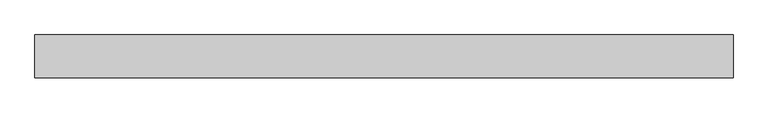
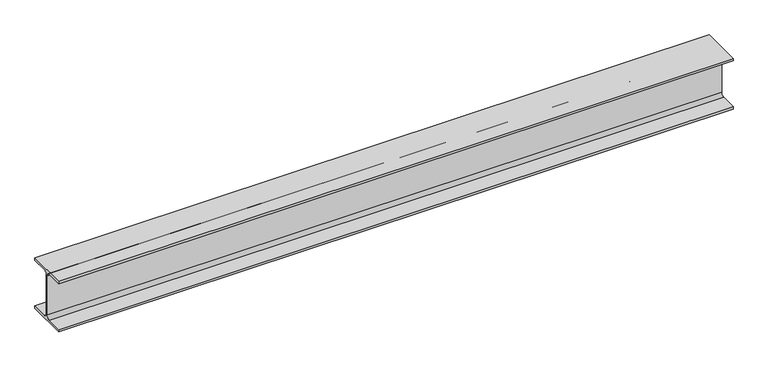
"""IFC4 building model written with IfcOpenShell, lengths in millimetres: beam geometry, 0912_Steel Framing_H-KSD3502 : H_SB_ASB_H-194x150x6x9."""

import ifcopenshell
import ifcopenshell.guid

model = None  # the IFC model being written
_history = None  # IfcOwnerHistory: only IFC2X3 demands one
_inside = {}  # id of a spatial element -> (the spatial element, [elements in it])
_under = {}  # id of a project, library or spatial element -> (it, [spatial elements below it])
_declared = {}  # id of a project -> (the project, [libraries it declares])
_typed = {}  # id of a type object -> (the type object, [elements of that type])
_made_of = {}  # id of a material, layer set ... -> (it, [elements and type objects made of it])


def new_model(schema):
    """Start an empty IFC model of exactly this schema.

    Asked for "IFC4X3", IfcOpenShell would pick the latest addendum, in which some entities
    have other attributes; the version numbers below select the first issue.
    IFC2X3 requires an IfcOwnerHistory on every rooted entity: one is made here for all.
    """
    global model, _history
    if schema == "IFC4X3":
        model = ifcopenshell.file(schema_version=(4, 3, 0, 0))
    else:
        model = ifcopenshell.file(schema=schema)
    _inside.clear()
    _under.clear()
    _declared.clear()
    _typed.clear()
    _made_of.clear()
    _history = None
    if model.schema == "IFC2X3":
        org = make("IfcOrganization", Name="unknown")
        user = make(
            "IfcPersonAndOrganization",
            ThePerson=make("IfcPerson", FamilyName="unknown"),
            TheOrganization=org,
        )
        app = make(
            "IfcApplication",
            ApplicationDeveloper=org,
            Version="unknown",
            ApplicationFullName="unknown",
            ApplicationIdentifier="unknown",
        )
        _history = make(
            "IfcOwnerHistory",
            OwningUser=user,
            OwningApplication=app,
            ChangeAction="ADDED",
            CreationDate=0,
        )
    return model


def make(cls, **values):
    """One entity of the class cls with the attributes given. An attribute that is None is left unset."""
    return model.create_entity(
        cls, **{name: value for name, value in values.items() if value is not None}
    )


def rooted(cls, **values):
    """An entity with a GlobalId (a new one), such as an element, a storey or a relation."""
    return make(cls, GlobalId=ifcopenshell.guid.new(), OwnerHistory=_history, **values)


def si_unit(unit_type, name, prefix=None):
    """IfcSIUnit, for example si_unit("LENGTHUNIT", "METRE", prefix="MILLI")."""
    return make("IfcSIUnit", UnitType=unit_type, Prefix=prefix, Name=name)


def assignment(units):
    """IfcUnitAssignment: the units of a project."""
    return None if units is None else make("IfcUnitAssignment", Units=units)


def point(xyz):
    """IfcCartesianPoint."""
    return None if xyz is None else make("IfcCartesianPoint", Coordinates=xyz)


def direction(xyz):
    """IfcDirection."""
    return None if xyz is None else make("IfcDirection", DirectionRatios=xyz)


def frame(location, z_axis=None, x_axis=None):
    """IfcAxis2Placement3D, a coordinate frame: its origin and axes. An axis left out is left unset."""
    return make(
        "IfcAxis2Placement3D",
        Location=point(location),
        Axis=direction(z_axis),
        RefDirection=direction(x_axis),
    )


def frame_2d(location, x_axis=None):
    """IfcAxis2Placement2D, a coordinate frame in the plane: its origin and x axis."""
    return make(
        "IfcAxis2Placement2D", Location=point(location), RefDirection=direction(x_axis)
    )


def origin():
    """The frame at (0, 0, 0) with its axes left unset."""
    return frame((0.0, 0.0, 0.0))


def place(relative_to, where):
    """IfcLocalPlacement: puts the frame where relative to a parent placement (None: the world)."""
    return make(
        "IfcLocalPlacement", PlacementRelTo=relative_to, RelativePlacement=where
    )


def context(
    kind, dimensions, precision=None, world=None, true_north=None, identifier=None
):
    """IfcGeometricRepresentationContext, for example the 3D "Model" context."""
    return make(
        "IfcGeometricRepresentationContext",
        ContextIdentifier=identifier,
        ContextType=kind,
        CoordinateSpaceDimension=dimensions,
        Precision=precision,
        WorldCoordinateSystem=world,
        TrueNorth=true_north,
    )


def project(units=None, contexts=None):
    """IfcProject with its units and contexts."""
    return rooted(
        "IfcProject",
        Name="project",
        RepresentationContexts=contexts,
        UnitsInContext=assignment(units),
    )


def spatial(cls, under=None, at=None, **own):
    """A site, building, storey or space (cls), placed at a placement, below another one or the project."""
    s = rooted(cls, ObjectPlacement=at, **own)
    if under is not None:
        _under.setdefault(under.id(), (under, []))[1].append(s)
    return s


def polyline(points):
    """IfcPolyline through the points."""
    return make("IfcPolyline", Points=[point(p) for p in points])


def circle_curve(where, radius):
    """IfcCircle in the frame where."""
    return make("IfcCircle", Position=where, Radius=radius)


def trimmed(basis, trim1, trim2, sense, master):
    """IfcTrimmedCurve: the piece of a basis curve between two trims."""
    return make(
        "IfcTrimmedCurve",
        BasisCurve=basis,
        Trim1=trim1,
        Trim2=trim2,
        SenseAgreement=sense,
        MasterRepresentation=master,
    )


def segment(curve, same_sense, transition):
    """IfcCompositeCurveSegment."""
    return make(
        "IfcCompositeCurveSegment",
        Transition=transition,
        SameSense=same_sense,
        ParentCurve=curve,
    )


def composite_curve(segments, self_intersect=None):
    """IfcCompositeCurve: segments joined end to end."""
    return make("IfcCompositeCurve", Segments=segments, SelfIntersect=self_intersect)


def outline(outer, holes=None, kind="AREA"):
    """IfcArbitraryClosedProfileDef: a profile drawn as a closed curve; with holes, ...WithVoids."""
    if holes is None:
        return make("IfcArbitraryClosedProfileDef", ProfileType=kind, OuterCurve=outer)
    return make(
        "IfcArbitraryProfileDefWithVoids",
        ProfileType=kind,
        OuterCurve=outer,
        InnerCurves=holes,
    )


def extrude(swept, where, along, depth):
    """IfcExtrudedAreaSolid: the profile swept, set in the frame where, extruded along a direction by depth."""
    return make(
        "IfcExtrudedAreaSolid",
        SweptArea=swept,
        Position=where,
        ExtrudedDirection=direction(along),
        Depth=depth,
    )


def shape(context_of_items, identifier, shape_type, items):
    """IfcShapeRepresentation: the items that make up one representation, for example the "Body"."""
    return make(
        "IfcShapeRepresentation",
        ContextOfItems=context_of_items,
        RepresentationIdentifier=identifier,
        RepresentationType=shape_type,
        Items=items,
    )


def source(mapping_origin, context_of_items, identifier, shape_type, items):
    """IfcRepresentationMap: a shape defined once, which mapped items show again and again."""
    return make(
        "IfcRepresentationMap",
        MappingOrigin=mapping_origin,
        MappedRepresentation=shape(context_of_items, identifier, shape_type, items),
    )


def transform(
    local_origin,
    x_axis=None,
    y_axis=None,
    z_axis=None,
    scale=None,
    scale2=None,
    scale3=None,
    uniform=True,
):
    """IfcCartesianTransformationOperator3D, or its non-uniform kind. x_axis, y_axis, z_axis: its Axis1, 2, 3."""
    if uniform:
        return make(
            "IfcCartesianTransformationOperator3D",
            Axis1=direction(x_axis),
            Axis2=direction(y_axis),
            LocalOrigin=point(local_origin),
            Scale=scale,
            Axis3=direction(z_axis),
        )
    return make(
        "IfcCartesianTransformationOperator3DnonUniform",
        Axis1=direction(x_axis),
        Axis2=direction(y_axis),
        LocalOrigin=point(local_origin),
        Scale=scale,
        Axis3=direction(z_axis),
        Scale2=scale2,
        Scale3=scale3,
    )


def mapped(mapping_source, mapping_target):
    """IfcMappedItem: shows the shape of a source again, moved by a transform."""
    return make(
        "IfcMappedItem", MappingSource=mapping_source, MappingTarget=mapping_target
    )


def made_of(thing, what):
    """Note that an element or type object is made of a material, layer set ...; save() writes the relation."""
    if what is not None:
        _made_of.setdefault(what.id(), (what, []))[1].append(thing)
    return thing


def element(
    cls,
    number,
    at=None,
    inside=None,
    cuts=None,
    type_object=None,
    material=None,
    context=None,
    identifier="Body",
    shape_type=None,
    held_by="IfcProductDefinitionShape",
    body=None,
    shapes=None,
    **own,
):
    """One element of the class cls, such as IfcWall. Its Tag is "e" and its number.

    at: its placement. inside: the storey or other place that contains it. cuts: it is an
    opening in that element (IfcRelVoidsElement). A single representation is given by context,
    identifier, shape_type and body (its items); several are given by shapes. held_by: the class
    of the entity that holds the representations. save() writes the other relations.
    """
    e = rooted(cls, Tag="e%d" % number, ObjectPlacement=at, **own)
    if body is not None:
        shapes = [shape(context, identifier, shape_type, body)]
    if shapes is not None:
        e.Representation = make(held_by, Representations=shapes)
    if inside is not None:
        _inside.setdefault(inside.id(), (inside, []))[1].append(e)
    if cuts is not None:
        rooted(
            "IfcRelVoidsElement", RelatingBuildingElement=cuts, RelatedOpeningElement=e
        )
    if type_object is not None:
        _typed.setdefault(type_object.id(), (type_object, []))[1].append(e)
    return made_of(e, material)


def aggregate(whole, parts):
    """IfcRelAggregates: a whole, such as a stair, and the parts it consists of."""
    return rooted("IfcRelAggregates", RelatingObject=whole, RelatedObjects=parts)


def save(model, path):
    """Write the relations noted so far, then the file.

    IfcRelAggregates (storeys below a building ...), IfcRelContainedInSpatialStructure (elements
    in a storey), IfcRelDefinesByType, IfcRelAssociatesMaterial and IfcRelDeclares: one each for
    every whole, place, type object, material and project.
    """
    for whole, parts in _under.values():
        aggregate(whole, parts)
    for where, things in _inside.values():
        rooted(
            "IfcRelContainedInSpatialStructure",
            RelatedElements=things,
            RelatingStructure=where,
        )
    for kind, things in _typed.values():
        rooted("IfcRelDefinesByType", RelatedObjects=things, RelatingType=kind)
    for what, things in _made_of.values():
        rooted("IfcRelAssociatesMaterial", RelatedObjects=things, RelatingMaterial=what)
    for by, libraries in _declared.values():
        rooted("IfcRelDeclares", RelatingContext=by, RelatedDefinitions=libraries)
    model.write(path)


def beam_288211e0(model_context):
    return source(origin(), model_context, "Body", "SweptSolid", [
        extrude(outline(composite_curve([segment(polyline([(75.0, -88.0), (75.0, -97.0), (-75.0, -97.0), (-75.0, -88.0), (-16.0, -88.0)]), True, "CONTINUOUS"), segment(trimmed(circle_curve(frame_2d((-16.0, -75.0)), 13.0), [point((-16.0, -88.0))], [point((-3.0, -75.0))], True, "CARTESIAN"), True, "CONTINUOUS"), segment(polyline([(-3.0, -75.0), (-3.0, 75.0)]), True, "CONTINUOUS"), segment(trimmed(circle_curve(frame_2d((-16.0, 75.0)), 13.0), [point((-3.0, 75.0))], [point((-16.0, 88.0))], True, "CARTESIAN"), True, "CONTINUOUS"), segment(polyline([(-16.0, 88.0), (-75.0, 88.0), (-75.0, 97.0), (75.0, 97.0), (75.0, 88.0), (16.0, 88.0)]), True, "CONTINUOUS"), segment(trimmed(circle_curve(frame_2d((16.0, 75.0)), 13.0), [point((16.0, 88.0))], [point((3.0, 75.0))], True, "CARTESIAN"), True, "CONTINUOUS"), segment(polyline([(3.0, 75.0), (3.0, -75.0)]), True, "CONTINUOUS"), segment(trimmed(circle_curve(frame_2d((16.0, -75.0)), 13.0), [point((3.0, -75.0))], [point((16.0, -88.0))], True, "CARTESIAN"), True, "CONTINUOUS"), segment(polyline([(16.0, -88.0), (75.0, -88.0)]), True, "CONTINUOUS")], self_intersect=False)), frame((-1200.0, 0.0, 0.0), z_axis=(1.0, 0.0, 0.0), x_axis=(0.0, 1.0, 0.0)), (0.0, 0.0, 1.0), 2448.0465428),
    ])


if __name__ == "__main__":
    model = new_model("IFC4")
    model_context = context("Model", 3, world=origin())
    ifc_project = project(units=[si_unit("LENGTHUNIT", "METRE", prefix="MILLI")], contexts=[model_context])
    site = spatial("IfcSite", under=ifc_project)
    building = spatial("IfcBuilding", under=site)
    placement = place(None, origin())
    beam_shape = beam_288211e0(model_context)
    element("IfcBeam", 1, ObjectType="0912_Steel Framing_H-KSD3502 : H_SB_ASB_H-194x150x6x9", at=placement, inside=building, context=model_context, shape_type="MappedRepresentation", body=[
        mapped(beam_shape, transform((0.0, 0.0, 0.0), x_axis=(1.0, 0.0, 0.0), y_axis=(0.0, 1.0, 0.0), z_axis=(0.0, 0.0, 1.0))),
    ])
    save(model, "model.ifc")

# Revit data of these elements
# Type "0912_Steel Framing_H-KSD3502 : H_SB_ASB_H-194x150x6x9"
#   H_WM Code_1 = "S01AA002-00001 | Main Steel Structure Fabrication Work | Shelter/Building | Medium Steel - Standard (90KG/M>Weight≥30KG/M) | Material: (   )"
#   H_WM Code_2 = "S03AA028-00001 | Main Steel Structure Erection Work | Shelter/Building | Medium Steel (90KG/M>Weight≥30KG/M) | Material: (   )"
#   H_WM Code_3 = "S01AA010-00001 | Main Steel Structure Fabrication Work | Shelter/Building | Steel Painting/Coating | for Non-Fireproofed Steel Surface, Surface Preparation, Primer, Second & Final Coat | Material: (   )"
#   H_Q'ty Cal Type Tag = "SB-Q2"
#   Width = 15.0 cm
#   Web Thickness = 0.6 cm
#   Web Fillet = 1.3 cm
#   Warping Constant = 43316.0 cm⁶
#   W = 0
#   Torsional Moment of Inertia = 8.622 cm⁴
#   Section Area = 39.01 cm²
#   Plastic Modulus weak axis = 104.0 cm³
#   Plastic Modulus strong axis = 309.0 cm³
#   Perimeter = 0.95 m²/m
#   Nominal Weight = 30.60 kgf/m
#   Moment of Inertia weak axis = 507.00 cm⁴
#   Moment of Inertia strong axis = 2690.00 cm⁴
#   Height = 19.4 cm
#   Flange Thickness = 0.9 cm
#   Elastic Modulus weak axis = 67.6 cm³
#   Elastic Modulus strong axis = 277.0 cm³
#   Centroid Vertical = 9.7 cm
#   Centroid Horizontal = 7.5 cm
#   Ix = 26900000
#   Length [instance default] = 1.5240 m
#   Zx = 309000
#   b = 0.1500 m
#   h = 0.1940 m
#   r = 0.0130 m
#   s = 0.0060 m
#   t = 0.0090 m
#   A = 0.003901 m²
#   Structural Material [instance default] = Steel, 45-345
#   Assembly Code = ""
# Element 1 (IfcBeam, "0912_Steel Framing_H-KSD3502 : H_SB_ASB_H-194x150x6x9")
#   Structural Material = none
# Materials
#   "Steel, 45-345": class "Metal", colour RGB 189 187 185, transparency 0, Description = "Steel 345 MPa", Cost = 0
